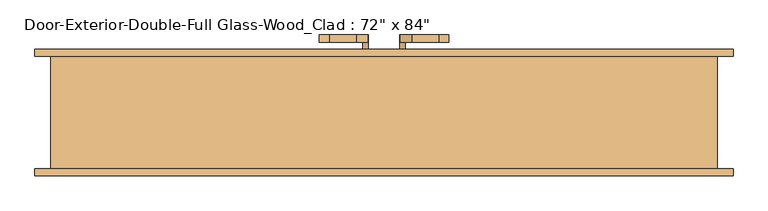
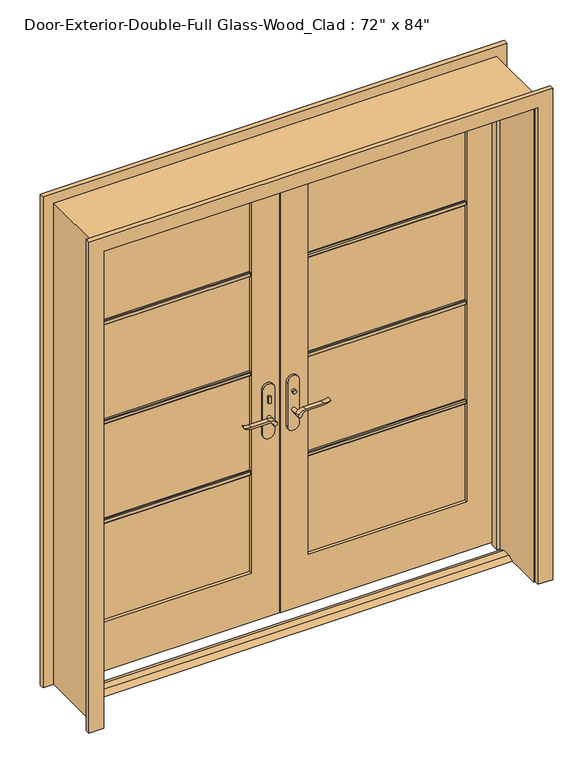
"""IFC4 building model written with IfcOpenShell, lengths in millimetres: door geometry."""

from ifc_helpers import new_model, si_unit, point, frame, frame_2d, origin, place, context, project, spatial, polyline, circle_curve, trimmed, segment, composite_curve, outline, extrude, faceted_brep, source, transform, mapped, element, save


def door_00124e33(model_context):
    return source(origin(), model_context, "Body", "SolidModel", [
        extrude(outline(polyline([(19.05, 12.7), (53.975, 12.7), (79.375, 0.0), (-6.35, 0.0), (19.05, 12.7)])), frame((-914.4, 0.0, 0.0), z_axis=(1.0, 0.0, 0.0), x_axis=(0.0, 1.0, 0.0)), (0.0, 0.0, 1.0), 1828.8),
        extrude(outline(polyline([(-47.4019111, 100.65), (-57.4019111, 100.65), (-57.4019111, 110.65), (-47.4019111, 110.65), (-47.4019111, 100.65)])), frame((0.0, 0.0, 981.9), z_axis=(0.0, 0.0, 1.0), x_axis=(1.0, 0.0, 0.0)), (0.0, 0.0, 1.0), 30.0),
        extrude(outline(composite_curve([segment(trimmed(circle_curve(frame_2d((996.9, -52.4019111)), 8.0), [point((996.9, -60.4019111))], [point((996.9, -44.4019111))], False, "CARTESIAN"), True, "CONTINUOUS"), segment(trimmed(circle_curve(frame_2d((996.9, -52.4019111)), 8.0), [point((996.9, -44.4019111))], [point((996.9, -60.4019111))], False, "CARTESIAN"), True, "CONTINUOUS")], self_intersect=False)), frame((0.0, 165.575, 0.0), z_axis=(0.0, 1.0, 0.0), x_axis=(0.0, 0.0, 1.0)), (0.0, 0.0, 1.0), 10.0),
        extrude(outline(composite_curve([segment(trimmed(circle_curve(frame_2d((897.1555521, -76.0694241)), 37.2832219), [point((919.0523287, -45.8937749))], [point((934.4, -77.7693445))], False, "CARTESIAN"), True, "CONTINUOUS"), segment(polyline([(934.4, -77.7693445), (934.4, -154.045502)]), True, "CONTINUOUS"), segment(trimmed(circle_curve(frame_2d((1017.6850638, -153.9791202)), 83.2850902), [point((934.4, -154.045502))], [point((939.4, -182.4019111))], True, "CARTESIAN"), True, "CONTINUOUS"), segment(polyline([(939.4, -182.4019111), (936.6135558, -182.4019111)]), True, "CONTINUOUS"), segment(trimmed(circle_curve(frame_2d((986.6709207, -150.4622499)), 59.3791355), [point((936.6135558, -182.4019111))], [point((927.4, -154.045502))], False, "CARTESIAN"), True, "CONTINUOUS"), segment(polyline([(927.4, -154.045502), (927.4, -77.7881013)]), True, "CONTINUOUS"), segment(trimmed(circle_curve(frame_2d((909.2738613, -77.7881013)), 18.1261387), [point((927.4, -77.7881013))], [point((914.4, -60.4019111))], True, "CARTESIAN"), True, "CONTINUOUS"), segment(trimmed(circle_curve(frame_2d((914.4, -52.4019111)), 8.0), [point((914.4, -60.4019111))], [point((919.0523287, -45.8937749))], False, "CARTESIAN"), True, "CONTINUOUS")], self_intersect=False)), frame((0.0, 60.65, 0.0), z_axis=(0.0, 1.0, 0.0), x_axis=(0.0, 0.0, 1.0)), (0.0, 0.0, 1.0), 20.0),
        extrude(outline(composite_curve([segment(trimmed(circle_curve(frame_2d((914.4, -52.4019111)), 8.0), [point((914.3999903, -60.4019111))], [point((919.0523287, -45.8937749))], False, "CARTESIAN"), True, "CONTINUOUS"), segment(trimmed(circle_curve(frame_2d((897.1555521, -76.0694241)), 37.2832219), [point((919.0523287, -45.8937749))], [point((934.4, -77.7693445))], False, "CARTESIAN"), True, "CONTINUOUS"), segment(polyline([(934.4, -77.7693445), (934.4, -154.045502)]), True, "CONTINUOUS"), segment(trimmed(circle_curve(frame_2d((1017.6850638, -153.9791202)), 83.2850902), [point((934.4, -154.045502))], [point((939.4, -182.4019111))], True, "CARTESIAN"), True, "CONTINUOUS"), segment(polyline([(939.4, -182.4019111), (936.6135558, -182.4019111)]), True, "CONTINUOUS"), segment(trimmed(circle_curve(frame_2d((986.6709207, -150.4622499)), 59.3791355), [point((936.6135558, -182.4019111))], [point((927.4, -154.045502))], False, "CARTESIAN"), True, "CONTINUOUS"), segment(polyline([(927.4, -154.045502), (927.4, -77.788099)]), True, "CONTINUOUS"), segment(trimmed(circle_curve(frame_2d((909.2738682, -77.788099)), 18.1261318), [point((927.4, -77.788099))], [point((914.3999903, -60.4019111))], True, "CARTESIAN"), True, "CONTINUOUS")], self_intersect=False)), frame((0.0, 195.575, 0.0), z_axis=(0.0, 1.0, 0.0), x_axis=(0.0, 0.0, 1.0)), (0.0, 0.0, 1.0), 20.0),
        extrude(outline(composite_curve([segment(trimmed(circle_curve(frame_2d((914.4, -52.4019111)), 8.0), [point((914.4, -60.4019111))], [point((914.4, -44.4019111))], False, "CARTESIAN"), True, "CONTINUOUS"), segment(trimmed(circle_curve(frame_2d((914.4, -52.4019111)), 8.0), [point((914.4, -44.4019111))], [point((914.4, -60.4019111))], False, "CARTESIAN"), True, "CONTINUOUS")], self_intersect=False)), frame((0.0, 80.65, 0.0), z_axis=(0.0, 1.0, 0.0), x_axis=(0.0, 0.0, 1.0)), (0.0, 0.0, 1.0), 30.0),
        extrude(outline(composite_curve([segment(trimmed(circle_curve(frame_2d((914.4, -52.4019111)), 8.0), [point((914.4, -60.4019111))], [point((914.4, -44.4019111))], False, "CARTESIAN"), True, "CONTINUOUS"), segment(trimmed(circle_curve(frame_2d((914.4, -52.4019111)), 8.0), [point((914.4, -44.4019111))], [point((914.4, -60.4019111))], False, "CARTESIAN"), True, "CONTINUOUS")], self_intersect=False)), frame((0.0, 165.575, 0.0), z_axis=(0.0, 1.0, 0.0), x_axis=(0.0, 0.0, 1.0)), (0.0, 0.0, 1.0), 30.0),
        extrude(outline(composite_curve([segment(polyline([(844.4, -27.4019111), (1039.4, -27.4019111)]), True, "CONTINUOUS"), segment(trimmed(circle_curve(frame_2d((1039.4, -52.4019111)), 25.0), [point((1039.4, -27.4019111))], [point((1039.4, -77.4019111))], False, "CARTESIAN"), True, "CONTINUOUS"), segment(polyline([(1039.4, -77.4019111), (844.4, -77.4019111)]), True, "CONTINUOUS"), segment(trimmed(circle_curve(frame_2d((844.4, -52.4019111)), 25.0), [point((844.4, -77.4019111))], [point((844.4, -27.4019111))], False, "CARTESIAN"), True, "CONTINUOUS")], self_intersect=False)), frame((0.0, 110.65, 0.0), z_axis=(0.0, 1.0, 0.0), x_axis=(0.0, 0.0, 1.0)), (0.0, 0.0, 1.0), 10.0),
        extrude(outline(composite_curve([segment(polyline([(844.4, -27.4019111), (1039.4, -27.4019111)]), True, "CONTINUOUS"), segment(trimmed(circle_curve(frame_2d((1039.4, -52.4019111)), 25.0), [point((1039.4, -27.4019111))], [point((1039.4, -77.4019111))], False, "CARTESIAN"), True, "CONTINUOUS"), segment(polyline([(1039.4, -77.4019111), (844.4, -77.4019111)]), True, "CONTINUOUS"), segment(trimmed(circle_curve(frame_2d((844.4, -52.4019111)), 25.0), [point((844.4, -77.4019111))], [point((844.4, -27.4019111))], False, "CARTESIAN"), True, "CONTINUOUS")], self_intersect=False)), frame((0.0, 155.575, 0.0), z_axis=(0.0, 1.0, 0.0), x_axis=(0.0, 0.0, 1.0)), (0.0, 0.0, 1.0), 10.0),
        extrude(outline(polyline([(47.3875, 175.575), (57.3875, 175.575), (57.3875, 165.575), (47.3875, 165.575), (47.3875, 175.575)])), frame((0.0, 0.0, 981.9), z_axis=(0.0, 0.0, 1.0), x_axis=(1.0, 0.0, 0.0)), (0.0, 0.0, 1.0), 30.0),
        extrude(outline(composite_curve([segment(trimmed(circle_curve(frame_2d((996.9, 52.3875)), 8.0), [point((996.9, 60.3875))], [point((996.9, 44.3875))], False, "CARTESIAN"), True, "CONTINUOUS"), segment(trimmed(circle_curve(frame_2d((996.9, 52.3875)), 8.0), [point((996.9, 44.3875))], [point((996.9, 60.3875))], False, "CARTESIAN"), True, "CONTINUOUS")], self_intersect=False)), frame((0.0, 100.65, 0.0), z_axis=(0.0, 1.0, 0.0), x_axis=(0.0, 0.0, 1.0)), (0.0, 0.0, 1.0), 10.0),
        extrude(outline(composite_curve([segment(trimmed(circle_curve(frame_2d((914.4, 52.3875)), 8.0), [point((919.0523287, 45.8793637))], [point((914.4, 60.3875))], False, "CARTESIAN"), True, "CONTINUOUS"), segment(trimmed(circle_curve(frame_2d((909.2738613, 77.7736901)), 18.1261387), [point((914.4, 60.3875))], [point((927.4, 77.7736901))], True, "CARTESIAN"), True, "CONTINUOUS"), segment(polyline([(927.4, 77.7736901), (927.4, 154.0310909)]), True, "CONTINUOUS"), segment(trimmed(circle_curve(frame_2d((986.6709207, 150.4478388)), 59.3791355), [point((927.4, 154.0310909))], [point((936.6135558, 182.3875))], False, "CARTESIAN"), True, "CONTINUOUS"), segment(polyline([(936.6135558, 182.3875), (939.4, 182.3875)]), True, "CONTINUOUS"), segment(trimmed(circle_curve(frame_2d((1017.6850638, 153.9647091)), 83.2850902), [point((939.4, 182.3875))], [point((934.4, 154.0310909))], True, "CARTESIAN"), True, "CONTINUOUS"), segment(polyline([(934.4, 154.0310909), (934.4, 77.7549333)]), True, "CONTINUOUS"), segment(trimmed(circle_curve(frame_2d((897.1555521, 76.0550129)), 37.2832219), [point((934.4, 77.7549333))], [point((919.0523287, 45.8793637))], False, "CARTESIAN"), True, "CONTINUOUS")], self_intersect=False)), frame((0.0, 195.575, 0.0), z_axis=(0.0, 1.0, 0.0), x_axis=(0.0, 0.0, 1.0)), (0.0, 0.0, 1.0), 20.0),
        extrude(outline(composite_curve([segment(trimmed(circle_curve(frame_2d((909.2738682, 77.7736878)), 18.1261318), [point((914.3999903, 60.3875))], [point((927.4, 77.7736878))], True, "CARTESIAN"), True, "CONTINUOUS"), segment(polyline([(927.4, 77.7736878), (927.4, 154.0310909)]), True, "CONTINUOUS"), segment(trimmed(circle_curve(frame_2d((986.6709207, 150.4478388)), 59.3791355), [point((927.4, 154.0310909))], [point((936.6135558, 182.3875))], False, "CARTESIAN"), True, "CONTINUOUS"), segment(polyline([(936.6135558, 182.3875), (939.4, 182.3875)]), True, "CONTINUOUS"), segment(trimmed(circle_curve(frame_2d((1017.6850638, 153.9647091)), 83.2850902), [point((939.4, 182.3875))], [point((934.4, 154.0310909))], True, "CARTESIAN"), True, "CONTINUOUS"), segment(polyline([(934.4, 154.0310909), (934.4, 77.7549333)]), True, "CONTINUOUS"), segment(trimmed(circle_curve(frame_2d((897.1555521, 76.0550129)), 37.2832219), [point((934.4, 77.7549333))], [point((919.0523287, 45.8793637))], False, "CARTESIAN"), True, "CONTINUOUS"), segment(trimmed(circle_curve(frame_2d((914.4, 52.3875)), 8.0), [point((919.0523287, 45.8793637))], [point((914.3999903, 60.3875))], False, "CARTESIAN"), True, "CONTINUOUS")], self_intersect=False)), frame((0.0, 60.65, 0.0), z_axis=(0.0, 1.0, 0.0), x_axis=(0.0, 0.0, 1.0)), (0.0, 0.0, 1.0), 20.0),
        extrude(outline(composite_curve([segment(trimmed(circle_curve(frame_2d((914.4, 52.3875)), 8.0), [point((914.4, 60.3875))], [point((914.4, 44.3875))], False, "CARTESIAN"), True, "CONTINUOUS"), segment(trimmed(circle_curve(frame_2d((914.4, 52.3875)), 8.0), [point((914.4, 44.3875))], [point((914.4, 60.3875))], False, "CARTESIAN"), True, "CONTINUOUS")], self_intersect=False)), frame((0.0, 165.575, 0.0), z_axis=(0.0, 1.0, 0.0), x_axis=(0.0, 0.0, 1.0)), (0.0, 0.0, 1.0), 30.0),
        extrude(outline(composite_curve([segment(trimmed(circle_curve(frame_2d((914.4, 52.3875)), 8.0), [point((914.4, 60.3875))], [point((914.4, 44.3875))], False, "CARTESIAN"), True, "CONTINUOUS"), segment(trimmed(circle_curve(frame_2d((914.4, 52.3875)), 8.0), [point((914.4, 44.3875))], [point((914.4, 60.3875))], False, "CARTESIAN"), True, "CONTINUOUS")], self_intersect=False)), frame((0.0, 80.65, 0.0), z_axis=(0.0, 1.0, 0.0), x_axis=(0.0, 0.0, 1.0)), (0.0, 0.0, 1.0), 30.0),
        extrude(outline(composite_curve([segment(trimmed(circle_curve(frame_2d((844.4, 52.3875)), 25.0), [point((844.4, 27.3875))], [point((844.4, 77.3875))], False, "CARTESIAN"), True, "CONTINUOUS"), segment(polyline([(844.4, 77.3875), (1039.4, 77.3875)]), True, "CONTINUOUS"), segment(trimmed(circle_curve(frame_2d((1039.4, 52.3875)), 25.0), [point((1039.4, 77.3875))], [point((1039.4, 27.3875))], False, "CARTESIAN"), True, "CONTINUOUS"), segment(polyline([(1039.4, 27.3875), (844.4, 27.3875)]), True, "CONTINUOUS")], self_intersect=False)), frame((0.0, 155.575, 0.0), z_axis=(0.0, 1.0, 0.0), x_axis=(0.0, 0.0, 1.0)), (0.0, 0.0, 1.0), 10.0),
        extrude(outline(composite_curve([segment(trimmed(circle_curve(frame_2d((844.4, 52.3875)), 25.0), [point((844.4, 27.3875))], [point((844.4, 77.3875))], False, "CARTESIAN"), True, "CONTINUOUS"), segment(polyline([(844.4, 77.3875), (1039.4, 77.3875)]), True, "CONTINUOUS"), segment(trimmed(circle_curve(frame_2d((1039.4, 52.3875)), 25.0), [point((1039.4, 77.3875))], [point((1039.4, 27.3875))], False, "CARTESIAN"), True, "CONTINUOUS"), segment(polyline([(1039.4, 27.3875), (844.4, 27.3875)]), True, "CONTINUOUS")], self_intersect=False)), frame((0.0, 110.65, 0.0), z_axis=(0.0, 1.0, 0.0), x_axis=(0.0, 0.0, 1.0)), (0.0, 0.0, 1.0), 10.0),
        extrude(outline(polyline([(134.62, 1578.371875), (134.62, 1559.321875), (128.27, 1559.321875), (125.095, 1562.496875), (125.095, 1575.196875), (128.27, 1578.371875), (134.62, 1578.371875)])), frame((120.65, 0.0, 0.0), z_axis=(1.0, 0.0, 0.0), x_axis=(0.0, 1.0, 0.0)), (0.0, 0.0, 1.0), 673.1),
        extrude(outline(polyline([(134.62, 1132.68125), (134.62, 1113.63125), (128.27, 1113.63125), (125.095, 1116.80625), (125.095, 1129.50625), (128.27, 1132.68125), (134.62, 1132.68125)])), frame((120.65, 0.0, 0.0), z_axis=(1.0, 0.0, 0.0), x_axis=(0.0, 1.0, 0.0)), (0.0, 0.0, 1.0), 673.1),
        extrude(outline(polyline([(134.62, 686.990625), (134.62, 667.940625), (128.27, 667.940625), (125.095, 671.115625), (125.095, 683.815625), (128.27, 686.990625), (134.62, 686.990625)])), frame((120.65, 0.0, 0.0), z_axis=(1.0, 0.0, 0.0), x_axis=(0.0, 1.0, 0.0)), (0.0, 0.0, 1.0), 673.1),
        extrude(outline(polyline([(141.605, 1578.371875), (147.955, 1578.371875), (151.13, 1575.196875), (151.13, 1562.496875), (147.955, 1559.321875), (141.605, 1559.321875), (141.605, 1578.371875)])), frame((-793.75, 0.0, 0.0), z_axis=(1.0, 0.0, 0.0), x_axis=(0.0, 1.0, 0.0)), (0.0, 0.0, 1.0), 673.1),
        extrude(outline(polyline([(141.605, 1132.68125), (147.955, 1132.68125), (151.13, 1129.50625), (151.13, 1116.80625), (147.955, 1113.63125), (141.605, 1113.63125), (141.605, 1132.68125)])), frame((-793.75, 0.0, 0.0), z_axis=(1.0, 0.0, 0.0), x_axis=(0.0, 1.0, 0.0)), (0.0, 0.0, 1.0), 673.1),
        extrude(outline(polyline([(141.605, 686.990625), (147.955, 686.990625), (151.13, 683.815625), (151.13, 671.115625), (147.955, 667.940625), (141.605, 667.940625), (141.605, 686.990625)])), frame((-793.75, 0.0, 0.0), z_axis=(1.0, 0.0, 0.0), x_axis=(0.0, 1.0, 0.0)), (0.0, 0.0, 1.0), 673.1),
        extrude(outline(polyline([(141.605, 1578.371875), (147.955, 1578.371875), (151.13, 1575.196875), (151.13, 1562.496875), (147.955, 1559.321875), (141.605, 1559.321875), (141.605, 1578.371875)])), frame((120.65, 0.0, 0.0), z_axis=(1.0, 0.0, 0.0), x_axis=(0.0, 1.0, 0.0)), (0.0, 0.0, 1.0), 673.1),
        extrude(outline(polyline([(141.605, 1132.68125), (147.955, 1132.68125), (151.13, 1129.50625), (151.13, 1116.80625), (147.955, 1113.63125), (141.605, 1113.63125), (141.605, 1132.68125)])), frame((120.65, 0.0, 0.0), z_axis=(1.0, 0.0, 0.0), x_axis=(0.0, 1.0, 0.0)), (0.0, 0.0, 1.0), 673.1),
        extrude(outline(polyline([(141.605, 686.990625), (147.955, 686.990625), (151.13, 683.815625), (151.13, 671.115625), (147.955, 667.940625), (141.605, 667.940625), (141.605, 686.990625)])), frame((120.65, 0.0, 0.0), z_axis=(1.0, 0.0, 0.0), x_axis=(0.0, 1.0, 0.0)), (0.0, 0.0, 1.0), 673.1),
        extrude(outline(polyline([(134.62, 1578.371875), (134.62, 1559.321875), (128.27, 1559.321875), (125.095, 1562.496875), (125.095, 1575.196875), (128.27, 1578.371875), (134.62, 1578.371875)])), frame((-793.75, 0.0, 0.0), z_axis=(1.0, 0.0, 0.0), x_axis=(0.0, 1.0, 0.0)), (0.0, 0.0, 1.0), 673.1),
        extrude(outline(polyline([(134.62, 1132.68125), (134.62, 1113.63125), (128.27, 1113.63125), (125.095, 1116.80625), (125.095, 1129.50625), (128.27, 1132.68125), (134.62, 1132.68125)])), frame((-793.75, 0.0, 0.0), z_axis=(1.0, 0.0, 0.0), x_axis=(0.0, 1.0, 0.0)), (0.0, 0.0, 1.0), 673.1),
        extrude(outline(polyline([(134.62, 686.990625), (134.62, 667.940625), (128.27, 667.940625), (125.095, 671.115625), (125.095, 683.815625), (128.27, 686.990625), (134.62, 686.990625)])), frame((-793.75, 0.0, 0.0), z_axis=(1.0, 0.0, 0.0), x_axis=(0.0, 1.0, 0.0)), (0.0, 0.0, 1.0), 673.1),
        extrude(outline(polyline([(0.0, 920.75), (0.0, 984.25), (2203.45, 984.25), (2203.45, -984.25), (0.0, -984.25), (0.0, -920.75), (2139.95, -920.75), (2139.95, 920.75), (0.0, 920.75)])), frame((0.0, 155.575, 0.0), z_axis=(0.0, 1.0, 0.0), x_axis=(0.0, 0.0, 1.0)), (0.0, 0.0, 1.0), 19.05),
        extrude(outline(polyline([(0.0, 920.75), (0.0, 984.25), (2203.45, 984.25), (2203.45, -984.25), (0.0, -984.25), (0.0, -920.75), (2139.95, -920.75), (2139.95, 920.75), (0.0, 920.75)])), frame((0.0, -180.975, 0.0), z_axis=(0.0, 1.0, 0.0), x_axis=(0.0, 0.0, 1.0)), (0.0, 0.0, 1.0), 19.05),
        extrude(outline(polyline([(12.7, 914.4), (2133.6, 914.4), (2133.6, 1.5875), (12.7, 1.5875), (12.7, 914.4)]), holes=[polyline([(2014.5375, 120.65), (2014.5375, 793.75), (231.775, 793.75), (231.775, 120.65), (2014.5375, 120.65)])]), frame((0.0, 120.65, 0.0), z_axis=(0.0, 1.0, 0.0), x_axis=(0.0, 0.0, 1.0)), (0.0, 0.0, 1.0), 34.925),
        extrude(outline(polyline([(2133.6, -914.4), (12.7, -914.4), (12.7, -1.6019111), (2133.6, -1.6019111), (2133.6, -914.4)]), holes=[polyline([(231.775, -793.75), (2014.5375, -793.75), (2014.5375, -120.65), (231.775, -120.65), (231.775, -793.75)])]), frame((0.0, 120.65, 0.0), z_axis=(0.0, 1.0, 0.0), x_axis=(0.0, 0.0, 1.0)), (0.0, 0.0, 1.0), 34.925),
        faceted_brep([(939.8, 155.575, 0.0), (939.8, -161.925, 0.0), (914.4, -161.925, 0.0), (914.4, 85.725, 0.0), (901.7, 85.725, 0.0), (901.7, 120.65, 0.0), (914.4, 120.65, 0.0), (914.4, 155.575, 0.0), (939.8, 155.575, 2159.0), (939.8, -161.925, 2159.0), (-939.8, -161.925, 2159.0), (-939.8, -161.925, 0.0), (-914.4, -161.925, 0.0), (-914.4, -161.925, 2133.6), (914.4, -161.925, 2133.6), (914.4, 85.725, 2133.6), (-914.4, 85.725, 2133.6), (-914.4, 85.725, 0.0), (-901.7, 85.725, 0.0), (-901.7, 85.725, 2120.9), (901.7, 85.725, 2120.9), (901.7, 120.65, 2120.9), (1.5875, 120.65, 2120.9), (-1.6019111, 120.65, 2120.9), (-901.7, 120.65, 2120.9), (-901.7, 120.65, 0.0), (-914.4, 120.65, 0.0), (-914.4, 120.65, 2133.6), (-1.6019111, 120.65, 2133.6), (1.5875, 120.65, 2133.6), (914.4, 120.65, 2133.6), (914.4, 155.575, 2133.6), (1.5875, 155.575, 2133.6), (-1.6019111, 155.575, 2133.6), (-914.4, 155.575, 2133.6), (-914.4, 155.575, 0.0), (-939.8, 155.575, 0.0), (-939.8, 155.575, 2159.0)], [[[0, 1, 2, 3, 4, 5, 6, 7]], [[1, 0, 8, 9]], [[2, 1, 9, 10, 11, 12, 13, 14]], [[3, 2, 14, 15]], [[4, 3, 15, 16, 17, 18, 19, 20]], [[5, 4, 20, 21]], [[6, 5, 21, 22, 23, 24, 25, 26, 27, 28, 29, 30]], [[7, 6, 30, 31]], [[0, 7, 31, 32, 33, 34, 35, 36, 37, 8]], [[9, 8, 37, 10]], [[14, 13, 16, 15]], [[20, 19, 24, 23, 22, 21]], [[31, 30, 29, 28, 27, 34, 33, 32]], [[12, 11, 36, 35, 26, 25, 18, 17]], [[11, 10, 37, 36]], [[13, 12, 17, 16]], [[19, 18, 25, 24]], [[27, 26, 35, 34]]]),
        extrude(outline(polyline([(793.75, 134.62), (120.65, 134.62), (120.65, 141.605), (793.75, 141.605), (793.75, 134.62)])), frame((0.0, 0.0, 231.775), z_axis=(0.0, 0.0, 1.0), x_axis=(1.0, 0.0, 0.0)), (0.0, 0.0, 1.0), 1782.7625),
        extrude(outline(polyline([(-120.65, 134.62), (-793.75, 134.62), (-793.75, 141.605), (-120.65, 141.605), (-120.65, 134.62)])), frame((0.0, 0.0, 231.775), z_axis=(0.0, 0.0, 1.0), x_axis=(1.0, 0.0, 0.0)), (0.0, 0.0, 1.0), 1782.7625),
    ])


if __name__ == "__main__":
    model = new_model("IFC4")
    model_context = context("Model", 3, world=origin())
    ifc_project = project(units=[si_unit("LENGTHUNIT", "METRE", prefix="MILLI")], contexts=[model_context])
    site = spatial("IfcSite", under=ifc_project)
    building = spatial("IfcBuilding", under=site)
    placement = place(None, origin())
    door_shape = door_00124e33(model_context)
    element("IfcDoor", 1, ObjectType="Door-Exterior-Double-Full Glass-Wood_Clad : 72\" x 84\"", at=placement, inside=building, context=model_context, shape_type="MappedRepresentation", body=[
        mapped(door_shape, transform((0.0, 0.0, 0.0), x_axis=(1.0, 0.0, 0.0), y_axis=(0.0, 1.0, 0.0), z_axis=(0.0, 0.0, 1.0))),
    ])
    save(model, "model.ifc")

# Revit data of these elements
# Type "Door-Exterior-Double-Full Glass-Wood_Clad : 72\" x 84\""
#   Type Mark = "24"
#   Assembly Code = "B2030100"
#   Analytic Construction = "French door, wood frame with double glass"
#   Top Rail = 0' - 4 11/16"
#   Threshold Offset [instance default] = 0' - 0 1/2"
#   Thickness = 0' - 1 3/8"
#   Thermal Resistance (R) = 1.9158 (h·ft²·°F)/BTU
#   Swing Angle [instance default] = 90.0000°
#   Stiles = 0' - 4 3/4"
#   Rough Width = 6' - 2"
#   Rough Height = 7' - 1"
#   Panel Width = 3' - 0"
#   Door Offset [instance default] = 0' - 0"
#   Height = 7' - 0"
#   Width = 6' - 0"
#   Heat Transfer Coefficient (U) = 0.5220 BTU/(h·ft²·°F)
#   Bottom Rail = 0' - 9 1/8"
#   Exterior Trim [instance default] = yes
#   Threshold [instance default] = yes
#   Show Grill [instance default] = yes
#   Function = 1
#   Trim Material = Clad - White
#   Threshold Material = Maple - Semigloss(Rotated)
#   Panel Material = Clad - White
#   Glazing = Glass, Clear Glazing
#   Frame Material = Clad - White
#   Door Handle Material = Aluminum
#   Visual Light Transmittance = 0
#   Solar Heat Gain Coefficient = 0
#   Wall Closure = (empty or 0)
#   Construction Type = (empty or 0)
# Element 1 (IfcDoor, "Door-Exterior-Double-Full Glass-Wood_Clad : 72\" x 84\"")
#   Materials on its faces: "Clad - White", "Aluminum", "Glass, Clear Glazing", "Maple - Semigloss(Rotated)"
# Materials
#   "Clad - White": class "Wood", colour RGB 245 245 243, transparency 0, Cost = 0
#   "Maple - Semigloss(Rotated)": class "Wood", colour RGB 196 161 118, transparency 0, Description = "Acer Saccharum", Cost = 0
#   "Glass, Clear Glazing": class "Glass", colour RGB 245 245 243, transparency 1, Description = "Clear glazing", Cost = 0
#   "Aluminum": class "Metal", colour RGB 244 245 246, transparency 0, Description = "Aluminum 6061", Cost = 0
